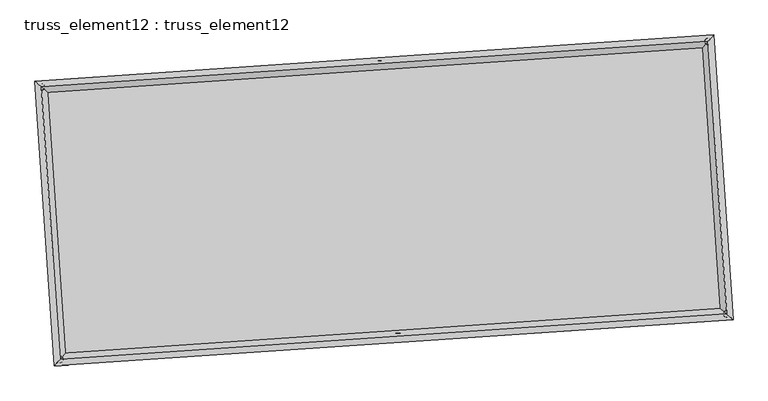
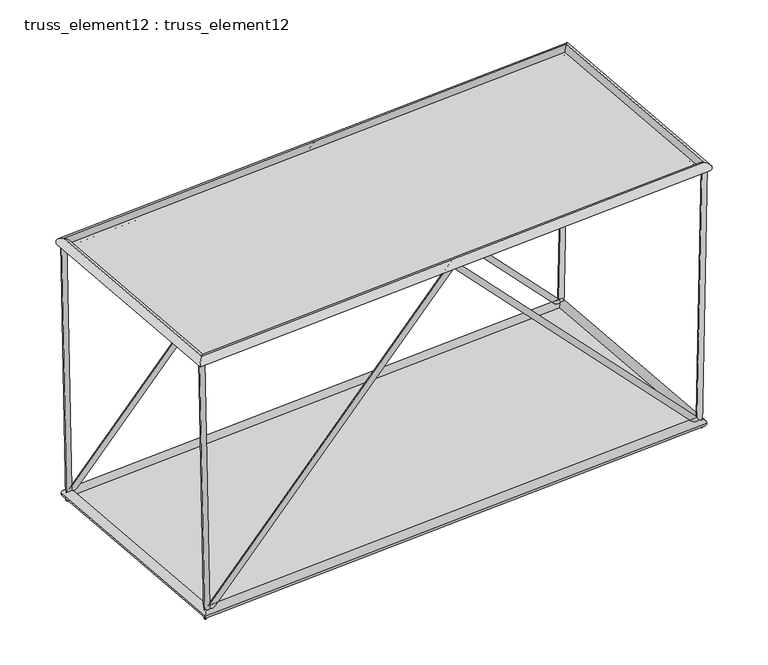
"""IFC4 building model written with IfcOpenShell, lengths in millimetres: plate geometry, truss_element12 : truss_element12."""

from ifc_helpers import new_model, si_unit, frame, origin, origin_with_axes, place, context, project, spatial, polyline, circle_curve, ellipse_curve, outline, extrude, source, transform, mapped, element, save
from ifc_brep_helpers import plane_surface, cylinder_surface, advanced_brep


def truss_element12_truss_element12_cebb5c17(model_context):
    return source(origin(), model_context, "Body", "SolidModel", [
        advanced_brep(
        [(-3767.1671851, 2269.2535853, 4999.9725392), (-3866.2496537, 2255.8937932, 4997.9279448), (-3667.4174306, 2276.0551419, 121.5871098), (-3761.5694522, 2263.0315382, -121.5871098), (1064.3618326, 2598.6971827, 5071.0530248), (1064.8004406, 2592.1233545, 4926.8210996), (5794.886864, 2921.2537021, 121.578348), (5889.874113, 2921.1267864, -121.578348), (5895.881521, 2928.1401439, 4999.9589337), (5995.8598643, 2928.3535519, 4997.8888311)],
        [
            (0, 1, circle_curve(frame((-3816.7084194, 2262.5736893, 4998.950242), z_axis=(-0.020442995593720103, -0.0013939301584342944, 0.9997900484050983), x_axis=(-0.13359837212382125, 0.9910346373676144, -0.001350001298501484)), 50.0)),
            (1, 0, circle_curve(frame((-3816.7084194, 2262.5736893, 4998.950242), z_axis=(-0.020442995593720103, -0.0013939301584342944, 0.9997900484050983), x_axis=(-0.13359837212382125, 0.9910346373676144, -0.001350001298501484)), 50.0)),
            (0, 2),
            (2, 3, ellipse_curve(frame((-3714.4934414, 2269.54334, 0.0), z_axis=(-0.9295196526265942, -0.06338041167761023, 0.3632852031070248), x_axis=(0.36244361517956775, 0.024713652341926906, 0.9316779814954776)), 130.7875297, 50.0)),
            (3, 1),
            (3, 2, ellipse_curve(frame((-3714.4934414, 2269.54334, 0.0), z_axis=(-0.9295196526265942, -0.06338041167761023, 0.3632852031070248), x_axis=(0.36244361517956775, 0.024713652341926906, 0.9316779814954776)), 130.7875297, 50.0)),
            (2, 4),
            (4, 5, ellipse_curve(frame((1064.5811366, 2595.4102686, 4998.9370622), z_axis=(-0.9976833938584647, -0.06802823807757291, 6.66567062485209e-05), x_axis=(-6.650228906135178e-05, -4.534538292208103e-06, -0.9999999977784416)), 72.2729929, 50.0)),
            (5, 3),
            (5, 4, ellipse_curve(frame((1064.5811366, 2595.4102686, 4998.9370622), z_axis=(-0.9976833938584647, -0.06802823807757291, 6.66567062485209e-05), x_axis=(-6.650228906135178e-05, -4.534538292208103e-06, -0.9999999977784416)), 72.2729929, 50.0)),
            (4, 6),
            (6, 7, ellipse_curve(frame((5842.3804885, 2921.1902443, 0.0), z_axis=(-0.9295901312719009, -0.06338521734851923, -0.36310398243970066), x_axis=(-0.3622628143287533, -0.024701324219198302, 0.9317486237910036)), 130.7681897, 50.0)),
            (7, 5),
            (7, 6, ellipse_curve(frame((5842.3804885, 2921.1902443, 0.0), z_axis=(-0.9295901312719009, -0.06338521734851923, -0.36310398243970066), x_axis=(-0.3622628143287533, -0.024701324219198302, 0.9317486237910036)), 130.7681897, 50.0)),
            (8, 9, circle_curve(frame((5945.8706927, 2928.2468479, 4998.9238824), z_axis=(0.020698040829792947, 0.0014113207235643172, 0.9997847764792299), x_axis=(-0.0021628361331172694, 0.999996726933573, -0.0013668438105636789)), 50.0)),
            (9, 8, circle_curve(frame((5945.8706927, 2928.2468479, 4998.9238824), z_axis=(0.020698040829792947, 0.0014113207235643172, 0.9997847764792299), x_axis=(-0.0021628361331172694, 0.999996726933573, -0.0013668438105636789)), 50.0)),
            (6, 8),
            (9, 7),
        ],
        [
            plane_surface(frame((-3816.7084194, 2312.5736407, 4999.0199531), z_axis=(-0.020442995593718667, -0.0013939301584386158, 0.9997900484050983), x_axis=(0.9997910201292846, -2.8502064444602113e-05, 0.020442975724613167))),
            cylinder_surface(frame((-3816.7084194, 2262.5736893, 4998.950242), z_axis=(-0.0204429955937201, -0.0013939301584342942, 0.9997900484050981), x_axis=(-0.13359837212382125, 0.9910346373676144, -0.001350001298501484)), 50.0),
            cylinder_surface(frame((-3714.4934414, 2269.54334, 0.0), z_axis=(-0.6902666987206841, -0.047066662236389376, -0.7220225854799657), x_axis=(-0.020420628738629147, 0.9987517974601704, -0.04558338504321424)), 50.0),
            cylinder_surface(frame((1064.5811366, 2595.4102686, 4998.9370622), z_axis=(-0.6901706602776501, -0.0470601137400352, 0.7221148145459193), x_axis=(-0.11534629536258453, 0.9922791770993238, -0.04557704291873413)), 50.0),
            plane_surface(frame((5945.8706927, 2878.2468977, 4998.9944636), z_axis=(0.02069804082979222, 0.0014113207235603308, 0.9997847764792298), x_axis=(0.999785772606216, -2.921783322129555e-05, -0.020698020207497326))),
            cylinder_surface(frame((5842.3804885, 2921.1902443, 0.0), z_axis=(-0.020698040829792947, -0.0014113207235643172, -0.9997847764792299), x_axis=(-0.0021628361331172694, 0.999996726933573, -0.0013668438105636789)), 50.0),
        ],
        [
            (0, [[1, 2]]),
            (1, [[-1, 3, 4, 5]]),
            (1, [[-2, -5, 6, -3]]),
            (2, [[-4, 7, 8, 9]]),
            (2, [[-6, -9, 10, -7]]),
            (3, [[-8, 11, 12, 13]]),
            (3, [[-10, -13, 14, -11]]),
            (4, [[15, 16]]),
            (5, [[-12, 17, -16, 18]]),
            (5, [[-14, -18, -15, -17]]),
        ],
    ),
        advanced_brep(
        [(-3495.0542322, -1721.479999, 4999.9725392), (-3594.1367008, -1734.8397911, 4997.9279448), (-3395.3044777, -1714.6784424, 121.5871098), (-3489.4564993, -1727.7020461, -121.5871098), (1336.4747855, -1392.0364016, 5071.0530248), (1336.9133936, -1398.6102298, 4926.8210996), (6066.9998169, -1069.4798822, 121.578348), (6161.9870659, -1069.6067979, -121.578348), (6167.9944739, -1062.5934404, 4999.9589337), (6267.9728172, -1062.3800324, 4997.8888311)],
        [
            (0, 1, circle_curve(frame((-3544.5954665, -1728.159895, 4998.950242), z_axis=(-0.0204429955937201, -0.001393930158434303, 0.9997900484050983), x_axis=(-0.1335983721238217, 0.9910346373676143, -0.001350001298501484)), 50.0)),
            (1, 0, circle_curve(frame((-3544.5954665, -1728.159895, 4998.950242), z_axis=(-0.0204429955937201, -0.001393930158434303, 0.9997900484050983), x_axis=(-0.1335983721238217, 0.9910346373676143, -0.001350001298501484)), 50.0)),
            (0, 2),
            (2, 3, ellipse_curve(frame((-3442.3804885, -1721.1902443, 0.0), z_axis=(-0.9295196526265942, -0.06338041167761047, 0.3632852031070248), x_axis=(0.36244361517956775, 0.024713652341926996, 0.9316779814954776)), 130.7875297, 50.0)),
            (3, 1),
            (3, 2, ellipse_curve(frame((-3442.3804885, -1721.1902443, 0.0), z_axis=(-0.9295196526265942, -0.06338041167761047, 0.3632852031070248), x_axis=(0.36244361517956775, 0.024713652341926996, 0.9316779814954776)), 130.7875297, 50.0)),
            (2, 4),
            (4, 5, ellipse_curve(frame((1336.6940895, -1395.3233157, 4998.9370622), z_axis=(-0.9976833938584648, -0.06802823807757319, 6.66567062488419e-05), x_axis=(-6.650228906135175e-05, -4.534538292198492e-06, -0.9999999977784417)), 72.2729929, 50.0)),
            (5, 3),
            (5, 4, ellipse_curve(frame((1336.6940895, -1395.3233157, 4998.9370622), z_axis=(-0.9976833938584648, -0.06802823807757319, 6.66567062488419e-05), x_axis=(-6.650228906135175e-05, -4.534538292198492e-06, -0.9999999977784417)), 72.2729929, 50.0)),
            (4, 6),
            (6, 7, ellipse_curve(frame((6114.4934414, -1069.54334, 0.0), z_axis=(-0.9295901312719014, -0.06338521734851954, -0.3631039824397004), x_axis=(-0.36226281432875257, -0.02470132421919832, 0.931748623791004)), 130.7681897, 50.0)),
            (7, 5),
            (7, 6, ellipse_curve(frame((6114.4934414, -1069.54334, 0.0), z_axis=(-0.9295901312719014, -0.06338521734851954, -0.3631039824397004), x_axis=(-0.36226281432875257, -0.02470132421919832, 0.931748623791004)), 130.7681897, 50.0)),
            (8, 9, circle_curve(frame((6217.9836456, -1062.4867364, 4998.9238824), z_axis=(0.020698040829793325, 0.0014113207235643879, 0.9997847764792299), x_axis=(-0.0021628361331172976, 0.999996726933573, -0.0013668438105637482)), 50.0)),
            (9, 8, circle_curve(frame((6217.9836456, -1062.4867364, 4998.9238824), z_axis=(0.020698040829793325, 0.0014113207235643879, 0.9997847764792299), x_axis=(-0.0021628361331172976, 0.999996726933573, -0.0013668438105637482)), 50.0)),
            (6, 8),
            (9, 7),
        ],
        [
            plane_surface(frame((-3544.5954665, -1678.1599436, 4999.0199531), z_axis=(-0.020442995593718667, -0.0013939301584386119, 0.9997900484050983), x_axis=(0.9997910201292846, -2.8502064444602113e-05, 0.020442975724613167))),
            cylinder_surface(frame((-3544.5954665, -1728.159895, 4998.950242), z_axis=(-0.020442995593720096, -0.0013939301584343028, 0.9997900484050981), x_axis=(-0.1335983721238217, 0.9910346373676143, -0.001350001298501484)), 50.0),
            cylinder_surface(frame((-3442.3804885, -1721.1902443, 0.0), z_axis=(-0.6902666987206841, -0.04706666223638955, -0.7220225854799657), x_axis=(-0.020420628738629217, 0.9987517974601704, -0.04558338504321442)), 50.0),
            cylinder_surface(frame((1336.6940895, -1395.3233157, 4998.9370622), z_axis=(-0.6901706602776495, -0.04706011374003534, 0.7221148145459199), x_axis=(-0.11534629536258498, 0.9922791770993238, -0.04557704291873424)), 50.0),
            plane_surface(frame((6217.9836456, -1112.4866866, 4998.9944636), z_axis=(0.020698040829792222, 0.0014113207235603214, 0.9997847764792299), x_axis=(0.999785772606216, -2.9217833220407372e-05, -0.020698020207497326))),
            cylinder_surface(frame((6114.4934414, -1069.54334, 0.0), z_axis=(-0.020698040829793325, -0.0014113207235643879, -0.9997847764792299), x_axis=(-0.0021628361331172976, 0.999996726933573, -0.0013668438105637482)), 50.0),
        ],
        [
            (0, [[1, 2]]),
            (1, [[-1, 3, 4, 5]]),
            (1, [[-2, -5, 6, -3]]),
            (2, [[-4, 7, 8, 9]]),
            (2, [[-6, -9, 10, -7]]),
            (3, [[-8, 11, 12, 13]]),
            (3, [[-10, -13, 14, -11]]),
            (4, [[15, 16]]),
            (5, [[-12, 17, -16, 18]]),
            (5, [[-14, -18, -15, -17]]),
        ],
    ),
        advanced_brep(
        [(-3544.602327, -1728.1674988, 4908.9502423), (-3544.5886059, -1728.1522913, 5088.9502417), (-3816.7005902, 2262.5670871, 5088.9502417), (-3816.7162486, 2262.5802914, 4908.9502423), (5945.8643159, 2928.2392771, 5088.9238821), (5945.8770694, 2928.2544187, 4908.9238827), (6217.9763001, -1062.4801013, 5088.9238821), (6217.990991, -1062.4933716, 4908.9238827)],
        [
            (0, 1, ellipse_curve(frame((-3544.5954665, -1728.159895, 4998.950242), z_axis=(-0.7535719234028931, 0.6573654662782613, 1.9048135841045667e-06), x_axis=(-0.6573654662755273, -0.7535719234052781, 1.9048135841050712e-06)), 127.2792206, 90.0)),
            (1, 2),
            (2, 3, ellipse_curve(frame((-3816.7084194, 2262.5736893, 4998.950242), z_axis=(-0.657365466275527, -0.7535719234052783, 1.904813584105534e-06), x_axis=(0.7535719234028931, -0.6573654662782611, -1.9048135841050305e-06)), 127.2792206, 90.0)),
            (3, 0),
            (1, 0, ellipse_curve(frame((-3544.5954665, -1728.159895, 4998.950242), z_axis=(-0.7535719234028931, 0.6573654662782613, 1.9048135841045667e-06), x_axis=(-0.6573654662755273, -0.7535719234052781, 1.9048135841050712e-06)), 127.2792206, 90.0)),
            (3, 2, ellipse_curve(frame((-3816.7084194, 2262.5736893, 4998.950242), z_axis=(-0.657365466275527, -0.7535719234052783, 1.904813584105534e-06), x_axis=(0.7535719234028931, -0.6573654662782611, -1.9048135841050305e-06)), 127.2792206, 90.0)),
            (2, 4),
            (4, 5, ellipse_curve(frame((5945.8706927, 2928.2468479, 4998.9238824), z_axis=(-0.7535719234028928, 0.6573654662782618, 1.9048135841054962e-06), x_axis=(-0.6573654662755274, -0.7535719234052779, 1.9048135841050684e-06)), 127.2792206, 90.0)),
            (5, 3),
            (5, 4, ellipse_curve(frame((5945.8706927, 2928.2468479, 4998.9238824), z_axis=(-0.7535719234028928, 0.6573654662782618, 1.9048135841054962e-06), x_axis=(-0.6573654662755274, -0.7535719234052779, 1.9048135841050684e-06)), 127.2792206, 90.0)),
            (4, 6),
            (6, 7, ellipse_curve(frame((6217.9836456, -1062.4867364, 4998.9238824), z_axis=(0.6573654662755276, 0.7535719234052778, -1.9048135841046055e-06), x_axis=(-0.7535719234028927, 0.6573654662782619, 1.9048135841050322e-06)), 127.2792206, 90.0)),
            (7, 5),
            (7, 6, ellipse_curve(frame((6217.9836456, -1062.4867364, 4998.9238824), z_axis=(0.6573654662755276, 0.7535719234052778, -1.9048135841046055e-06), x_axis=(-0.7535719234028927, 0.6573654662782619, 1.9048135841050322e-06)), 127.2792206, 90.0)),
            (6, 1),
            (0, 7),
        ],
        [
            cylinder_surface(frame((-3544.5954665, -1728.159895, 4998.950242), z_axis=(0.06802823822869425, -0.9976833960748771, 0.0), x_axis=(-0.9976833927370898, -0.06802823800110322, 8.179899131489945e-05)), 90.0),
            cylinder_surface(frame((-3816.7084194, 2262.5736893, 4998.950242), z_axis=(-0.9976833960712573, -0.06802823822844584, 2.6938132044341946e-06), x_axis=(-0.068028237803244, 0.9976833929678073, 7.9105178118894e-05)), 90.0),
            cylinder_surface(frame((5945.8706927, 2928.2468479, 4998.9238824), z_axis=(-0.06802823822869297, 0.9976833960748774, 0.0), x_axis=(0.9976833931622919, 0.06802823803009485, 7.641136492288858e-05)), 90.0),
            cylinder_surface(frame((6217.9836456, -1062.4867364, 4998.9238824), z_axis=(0.9976833960712573, 0.06802823822844561, -2.693813204433539e-06), x_axis=(0.06802823822844561, -0.9976833929388144, 7.910517811889402e-05)), 90.0),
        ],
        [
            (0, [[1, 2, 3, 4]]),
            (0, [[5, -4, 6, -2]]),
            (1, [[-3, 7, 8, 9]]),
            (1, [[-6, -9, 10, -7]]),
            (2, [[-8, 11, 12, 13]]),
            (2, [[-10, -13, 14, -11]]),
            (3, [[-12, 15, -1, 16]]),
            (3, [[-14, -16, -5, -15]]),
        ],
    ),
        advanced_brep(
        [(-3358.7115243, -1625.2761972, 0.0), (-3526.0494527, -1817.1042913, 0.0), (-3810.4074885, 2353.2123043, 0.0), (-3618.5793943, 2185.8743758, 0.0), (5926.0494527, 3017.1042913, 0.0), (5758.7115243, 2825.2761972, 0.0), (6210.4074885, -1153.2123043, 0.0), (6018.5793943, -985.8743758, 0.0)],
        [
            (0, 1, ellipse_curve(frame((-3442.3804885, -1721.1902443, 0.0), z_axis=(-0.7535719234054586, 0.65736546627808, 0.0), x_axis=(-0.65736546627808, -0.7535719234054588, 0.0)), 127.2792206, 90.0)),
            (1, 2),
            (2, 3, ellipse_curve(frame((-3714.4934414, 2269.54334, 0.0), z_axis=(-0.6573654662780802, -0.7535719234054584, 0.0), x_axis=(0.7535719234054583, -0.6573654662780802, 0.0)), 127.2792206, 90.0)),
            (3, 0),
            (1, 0, ellipse_curve(frame((-3442.3804885, -1721.1902443, 0.0), z_axis=(-0.7535719234054586, 0.65736546627808, 0.0), x_axis=(-0.65736546627808, -0.7535719234054588, 0.0)), 127.2792206, 90.0)),
            (3, 2, ellipse_curve(frame((-3714.4934414, 2269.54334, 0.0), z_axis=(-0.6573654662780802, -0.7535719234054584, 0.0), x_axis=(0.7535719234054583, -0.6573654662780802, 0.0)), 127.2792206, 90.0)),
            (2, 4),
            (4, 5, ellipse_curve(frame((5842.3804885, 2921.1902443, 0.0), z_axis=(-0.7535719234054581, 0.6573654662780807, 0.0), x_axis=(-0.6573654662780806, -0.753571923405458, 0.0)), 127.2792206, 90.0)),
            (5, 3),
            (5, 4, ellipse_curve(frame((5842.3804885, 2921.1902443, 0.0), z_axis=(-0.7535719234054581, 0.6573654662780807, 0.0), x_axis=(-0.6573654662780806, -0.753571923405458, 0.0)), 127.2792206, 90.0)),
            (4, 6),
            (6, 7, ellipse_curve(frame((6114.4934414, -1069.54334, 0.0), z_axis=(0.6573654662780805, 0.7535719234054582, 0.0), x_axis=(-0.7535719234054582, 0.6573654662780806, 0.0)), 127.2792206, 90.0)),
            (7, 5),
            (7, 6, ellipse_curve(frame((6114.4934414, -1069.54334, 0.0), z_axis=(0.6573654662780805, 0.7535719234054582, 0.0), x_axis=(-0.7535719234054582, 0.6573654662780806, 0.0)), 127.2792206, 90.0)),
            (6, 1),
            (0, 7),
        ],
        [
            cylinder_surface(frame((-3442.3804885, -1721.1902443, 0.0), z_axis=(0.06802823822870284, -0.9976833960748764, 0.0), x_axis=(-0.9976833960748764, -0.06802823822870284, 0.0)), 90.0),
            cylinder_surface(frame((-3714.4934414, 2269.54334, 0.0), z_axis=(-0.9976833960748765, -0.06802823822870127, 0.0), x_axis=(-0.06802823822870127, 0.9976833960748765, 0.0)), 90.0),
            cylinder_surface(frame((5842.3804885, 2921.1902443, 0.0), z_axis=(-0.06802823822870158, 0.9976833960748765, 0.0), x_axis=(0.9976833960748765, 0.06802823822870158, 0.0)), 90.0),
            cylinder_surface(frame((6114.4934414, -1069.54334, 0.0), z_axis=(0.9976833960748767, 0.06802823822870163, 0.0), x_axis=(0.06802823822870163, -0.9976833960748767, 0.0)), 90.0),
        ],
        [
            (0, [[1, 2, 3, 4]]),
            (0, [[5, -4, 6, -2]]),
            (1, [[-3, 7, 8, 9]]),
            (1, [[-6, -9, 10, -7]]),
            (2, [[-8, 11, 12, 13]]),
            (2, [[-10, -13, 14, -11]]),
            (3, [[-12, 15, -1, 16]]),
            (3, [[-14, -16, -5, -15]]),
        ],
    ),
        extrude(outline(polyline([(-3442.3804885, -1721.1902443), (-3714.4934414, 2269.54334), (5842.3804885, 2921.1902443), (6114.4934414, -1069.54334), (-3442.3804885, -1721.1902443)])), origin_with_axes(), (0.0, 0.0, 1.0), 20.0),
        extrude(outline(polyline([(-1999.9999999, 4892.6238276), (2000.0000001, 4892.6238276), (2000.0, -4892.6238276), (-2000.0, -4892.6238276), (-1999.9999999, 4892.6238276)])), frame((1200.6376131, 600.0434764, 4998.9370622), z_axis=(2.6875727061909235e-06, 1.832553664148525e-07, 0.9999999999963718), x_axis=(-0.0680282382287029, 0.9976833960748764, 0.0)), (0.0, 0.0, 1.0), 20.0),
    ])


if __name__ == "__main__":
    model = new_model("IFC4")
    model_context = context("Model", 3, world=origin())
    ifc_project = project(units=[si_unit("LENGTHUNIT", "METRE", prefix="MILLI")], contexts=[model_context])
    site = spatial("IfcSite", under=ifc_project)
    building = spatial("IfcBuilding", under=site)
    placement = place(None, origin())
    truss_element12_truss_element12_shape = truss_element12_truss_element12_cebb5c17(model_context)
    element("IfcPlate", 1, ObjectType="truss_element12 : truss_element12", at=placement, inside=building, context=model_context, shape_type="MappedRepresentation", body=[
        mapped(truss_element12_truss_element12_shape, transform((0.0, 0.0, 0.0), x_axis=(1.0, 0.0, 0.0), y_axis=(0.0, 1.0, 0.0), z_axis=(0.0, 0.0, 1.0))),
    ])
    save(model, "model.ifc")

# Revit data of these elements
# Type "truss_element12 : truss_element12"
#   steellbar1 = 90 mm
#   steelbar2 = 50 mm
#   offset1 = 5000 mm
#   M = Default Roof
# Element 1 (IfcPlate, "truss_element12 : truss_element12")
#   Materials on its faces: "Default Roof"
# Materials
#   "Default Roof": class "Miscellaneous", colour RGB 0 127 0, transparency 0, Comments = "Rendering appearance not upgraded Rendering appearance not upgraded ", Cost = 0
